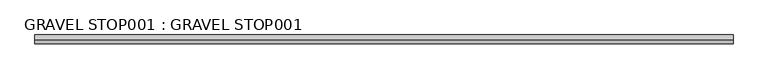
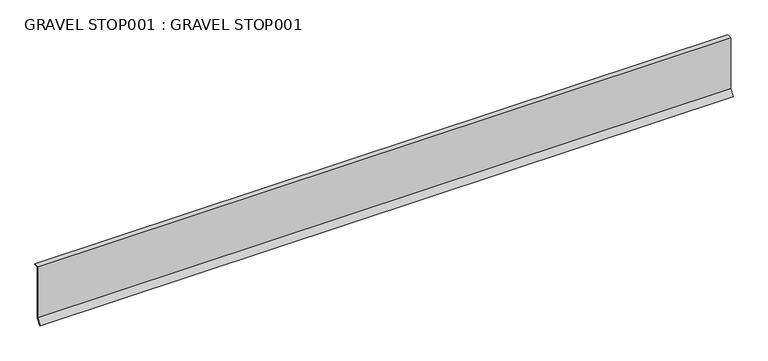
"""IFC4 building model written with IfcOpenShell, lengths in millimetres: proxy geometry, GRAVEL STOP001 : GRAVEL STOP001."""

from ifc_helpers import new_model, si_unit, frame, origin, place, context, project, spatial, polyline, outline, extrude, source, transform, mapped, element, save


def gravel_stop001_gravel_stop001_6aa894b6(model_context):
    return source(origin(), model_context, "Body", "SweptSolid", [
        extrude(outline(polyline([(-5588.2594715, 40065.903984), (-5575.6959005, 40081.6491197), (-5575.6959005, 40238.3989826), (-5562.5168708, 40238.3989826), (-5562.5168708, 40236.9878716), (-5574.2847895, 40236.9878716), (-5574.2847895, 40081.1551279), (-5587.1564679, 40065.0238605), (-5588.2594715, 40065.903984)])), frame((12382.7678845, 0.0, 0.0), z_axis=(1.0, 0.0, 0.0), x_axis=(0.0, 1.0, 0.0)), (0.0, 0.0, 1.0), 2000.25),
    ])


if __name__ == "__main__":
    model = new_model("IFC4")
    model_context = context("Model", 3, world=origin())
    ifc_project = project(units=[si_unit("LENGTHUNIT", "METRE", prefix="MILLI")], contexts=[model_context])
    site = spatial("IfcSite", under=ifc_project)
    building = spatial("IfcBuilding", under=site)
    placement = place(None, origin())
    gravel_stop001_gravel_stop001_shape = gravel_stop001_gravel_stop001_6aa894b6(model_context)
    element("IfcBuildingElementProxy", 1, Name="GRAVEL STOP001 : GRAVEL STOP001", ObjectType="GRAVEL STOP001 : GRAVEL STOP001", at=placement, inside=building, context=model_context, shape_type="MappedRepresentation", body=[
        mapped(gravel_stop001_gravel_stop001_shape, transform((0.0, 0.0, 0.0), x_axis=(1.0, 0.0, 0.0), y_axis=(0.0, 1.0, 0.0), z_axis=(0.0, 0.0, 1.0))),
    ])
    save(model, "model.ifc")

# Revit data of these elements
# Type "GRAVEL STOP001 : GRAVEL STOP001"
#   NameOverride = "GRAVEL STOP001"
# Element 1 (IfcBuildingElementProxy, "GRAVEL STOP001 : GRAVEL STOP001")
#   Materials on its faces: "GRAVEL STOP REQUIRED WITH GRAVEL SURFACE SYSTEMS"
# Materials
#   "GRAVEL STOP REQUIRED WITH GRAVEL SURFACE SYSTEMS": class "Unassigned", colour RGB 170 170 127, transparency 0
